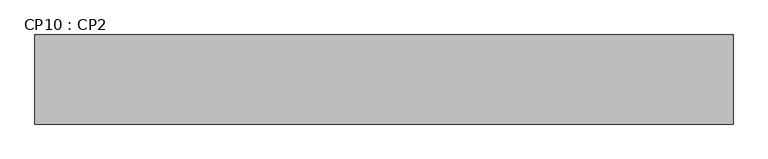
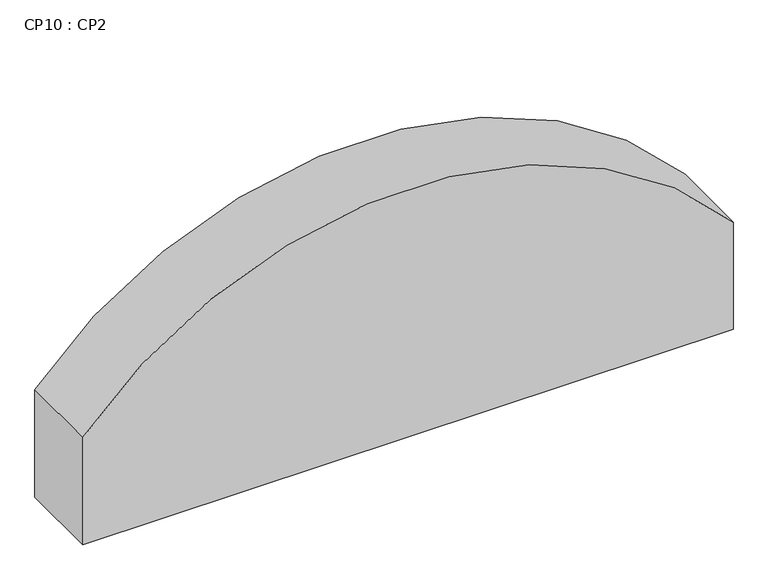
"""IFC4 building model written with IfcOpenShell, lengths in millimetres: beam geometry, CP10 : CP2."""

from ifc_helpers import new_model, si_unit, frame, origin, place, context, project, spatial, circle_curve, source, transform, mapped, element, save
from ifc_brep_helpers import plane_surface, cylinder_surface, advanced_brep


def cp10_cp2_f1d95e30(model_context):
    return source(origin(), model_context, "Body", "AdvancedBrep", [
        advanced_brep(
        [(45183.2245512, -100.2551788, 14620.0), (40483.2245513, -100.2551788, 14620.0), (40483.22455, -100.2551788, 13800.0), (45183.2245506, -100.2551788, 13800.0), (40483.2245513, 499.7448212, 14620.0), (45183.2245512, 499.7448212, 14620.0), (45183.2245506, 499.7448212, 13800.0), (40483.22455, 499.7448212, 13800.0)],
        [
            (0, 1, circle_curve(frame((42833.2245513, -100.2551788, 12603.8185575), z_axis=(0.0, -1.0, 0.0), x_axis=(0.0, 0.0, -1.0)), 3096.3668402)),
            (1, 2),
            (2, 3),
            (3, 0),
            (4, 5, circle_curve(frame((42833.2245513, 499.7448212, 12603.8185575), z_axis=(0.0, 1.0, 0.0), x_axis=(0.0, 0.0, -1.0)), 3096.3668402)),
            (5, 6),
            (6, 7),
            (7, 4),
            (2, 7),
            (6, 3),
            (0, 5),
            (4, 1),
        ],
        [
            plane_surface(frame((45333.2245515, -100.2551788, 13800.0), z_axis=(0.0, -1.0, 0.0), x_axis=(0.0, 0.0, 1.0))),
            plane_surface(frame((45333.2245515, 499.7448212, 13800.0), z_axis=(0.0, 1.0, 0.0), x_axis=(0.0, 0.0, -1.0))),
            plane_surface(frame((40333.2245516, -100.2551788, 13800.0), z_axis=(0.0, 0.0, -1.0), x_axis=(0.0, 1.0, 0.0))),
            cylinder_surface(frame((42833.2245513, 20099.7448193, 12603.8185575), z_axis=(0.0, 1.0, 0.0), x_axis=(0.0, 0.0, -1.0)), 3096.3668402),
            plane_surface(frame((40483.22455, 18587.0448193, 14620.0), z_axis=(-1.0, 0.0, 0.0), x_axis=(0.0, -1.0, 0.0))),
            plane_surface(frame((45183.2245506, 18587.0448193, 13800.0), z_axis=(1.0, 0.0, 0.0), x_axis=(0.0, -1.0, 0.0))),
        ],
        [
            (0, [[1, 2, 3, 4]]),
            (1, [[5, 6, 7, 8]]),
            (2, [[9, -7, 10, -3]]),
            (3, [[-1, 11, -5, 12]]),
            (4, [[-2, -12, -8, -9]]),
            (5, [[-4, -10, -6, -11]]),
        ],
    ),
    ])


if __name__ == "__main__":
    model = new_model("IFC4")
    model_context = context("Model", 3, world=origin())
    ifc_project = project(units=[si_unit("LENGTHUNIT", "METRE", prefix="MILLI")], contexts=[model_context])
    site = spatial("IfcSite", under=ifc_project)
    building = spatial("IfcBuilding", under=site)
    placement = place(None, origin())
    cp10_cp2_shape = cp10_cp2_f1d95e30(model_context)
    element("IfcBeam", 1, ObjectType="CP10 : CP2", at=placement, inside=building, context=model_context, shape_type="MappedRepresentation", body=[
        mapped(cp10_cp2_shape, transform((0.0, 0.0, 0.0), x_axis=(1.0, 0.0, 0.0), y_axis=(0.0, 1.0, 0.0), z_axis=(0.0, 0.0, 1.0))),
    ])
    save(model, "model.ifc")
